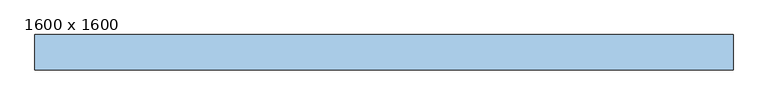
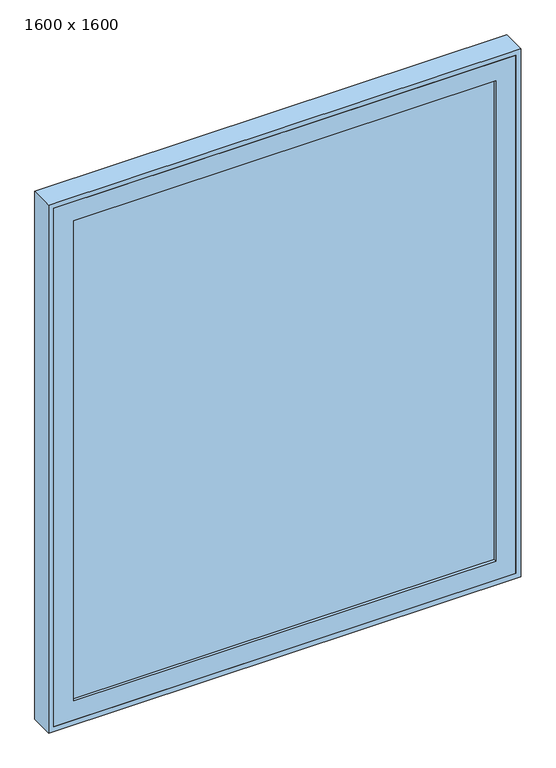
"""IFC4 building model written with IfcOpenShell, lengths in millimetres: window geometry, Aluprof_MB-79N-SI_E_Alu_Window-1sash-FIX_ENG_R-00206 : 1600 x 1600."""

from ifc_helpers import new_model, si_unit, frame, origin, place, context, project, spatial, polyline, outline, extrude, faceted_brep, source, transform, mapped, element, save


def window_1600_x_1600_1d4bee44(model_context):
    return source(origin(), model_context, "Body", "SolidModel", [
        faceted_brep([(-619.5, -58.5, 2315.5), (-619.5, -58.5, 826.5), (-619.5, -45.0, 826.5), (-619.5, -45.0, 2315.5), (-675.0, -45.0, 2371.0), (-675.0, -45.0, 771.0), (-675.0, -115.0, 771.0), (-675.0, -115.0, 2371.0), (619.5, -58.5, 826.5), (619.5, -45.0, 826.5), (675.0, -45.0, 771.0), (675.0, -115.0, 771.0), (619.5, -58.5, 2315.5), (619.5, -45.0, 2315.5), (675.0, -45.0, 2371.0), (675.0, -115.0, 2371.0), (-635.5, -58.5, 2331.5), (-635.5, -58.5, 810.5), (635.5, -58.5, 810.5), (635.5, -58.5, 2331.5), (-635.5, -106.5, 2331.5), (-635.5, -106.5, 810.5), (635.5, -106.5, 810.5), (635.5, -106.5, 2331.5), (-616.5, -106.5, 2312.5), (-616.5, -106.5, 829.5), (616.5, -106.5, 829.5), (616.5, -106.5, 2312.5), (-616.5, -115.0, 2312.5), (-616.5, -115.0, 829.5), (616.5, -115.0, 829.5), (616.5, -115.0, 2312.5)], [[[0, 1, 2, 3]], [[4, 5, 6, 7]], [[1, 8, 9, 2]], [[5, 10, 11, 6]], [[8, 12, 13, 9]], [[10, 14, 15, 11]], [[16, 17, 18, 19], [1, 0, 12, 8]], [[12, 0, 3, 13]], [[5, 4, 14, 10], [3, 2, 9, 13]], [[14, 4, 7, 15]], [[20, 21, 17, 16]], [[21, 22, 18, 17]], [[22, 23, 19, 18]], [[21, 20, 23, 22], [24, 25, 26, 27]], [[23, 20, 16, 19]], [[28, 29, 25, 24]], [[29, 30, 26, 25]], [[30, 31, 27, 26]], [[7, 6, 11, 15], [29, 28, 31, 30]], [[31, 28, 24, 27]]]),
        extrude(outline(polyline([(635.5, -58.5), (635.5, -106.5), (-635.5, -106.5), (-635.5, -58.5), (635.5, -58.5)])), frame((0.0, 0.0, 810.5), z_axis=(0.0, 0.0, 1.0), x_axis=(1.0, 0.0, 0.0)), (0.0, 0.0, 1.0), 1521.0),
        extrude(outline(polyline([(2386.0, -690.0), (756.0, -690.0), (756.0, 690.0), (2386.0, 690.0), (2386.0, -690.0)]), holes=[polyline([(771.0, -675.0), (2371.0, -675.0), (2371.0, 675.0), (771.0, 675.0), (771.0, -675.0)])]), frame((0.0, -115.0, 0.0), z_axis=(0.0, 1.0, 0.0), x_axis=(0.0, 0.0, 1.0)), (0.0, 0.0, 1.0), 70.0),
    ])


if __name__ == "__main__":
    model = new_model("IFC4")
    model_context = context("Model", 3, world=origin())
    ifc_project = project(units=[si_unit("LENGTHUNIT", "METRE", prefix="MILLI")], contexts=[model_context])
    site = spatial("IfcSite", under=ifc_project)
    building = spatial("IfcBuilding", under=site)
    placement = place(None, origin())
    window_1600_x_1600_shape = window_1600_x_1600_1d4bee44(model_context)
    element("IfcWindow", 1, ObjectType="Aluprof_MB-79N-SI_E_Alu_Window-1sash-FIX_ENG_R-00206 : 1600 x 1600", at=placement, inside=building, context=model_context, shape_type="MappedRepresentation", body=[
        mapped(window_1600_x_1600_shape, transform((0.0, 0.0, 0.0), x_axis=(1.0, 0.0, 0.0), y_axis=(0.0, 1.0, 0.0), z_axis=(0.0, 0.0, 1.0))),
    ])
    save(model, "model.ifc")

# Revit data of these elements
# Type "Aluprof_MB-79N-SI_E_Alu_Window-1sash-FIX_ENG_R-00206 : 1600 x 1600"
#   Type Mark = "58"
#   Water resistance = "Class E1950, EN 12208"
#   Uniclass2015Version = "v1.6"
#   Uniclass2015Reference = "Pr_30_59_98_02"
#   Uniclass2015Description = "Aluminium window units"
#   URL = "https://aluprof.eu/"
#   Resistance to wind load = "Class C5, EN 12210"
#   Product page URL = "https://aluprof.eu/architekci/katalog-dla-architektow/systemy-okienno-drzwiowe/mb-79n-si-system-okienno-drzwiowy-z-izolacja-termiczna#/materialy/ogolne-informacje"
#   Operation = "SinglePanel"
#   Opening type = "FIX"
#   NBSReference = "45-25-99/310"
#   NBSDescription = "Aluminium window units"
#   Model = "MB-79N SI"
#   Manufacturer = "ALUPROF S.A."
#   Insert type = "SI"
#   IfcExportType = "NOTDEFINED"
#   IfcExportAs = "IfcWindowType"
#   Glazing construction = "6/16/4/16/6"
#   Description = "Single fixed window"
#   Content of the recyclate in the material = "70.7%"
#   COBie.Type.WarrantyDurationParts = ""
#   COBie.Type.Name = ""
#   COBie.Type.Manufacturer = "ALUPROF SA"
#   COBie.Space.Name = ""
#   COBie.Floor.Name = ""
#   COBie.Facility.Name = ""
#   COBie.CreatedOn = ""
#   COBie.CreatedBy = "aluprof.eu"
#   COBie.Component.WarrantyStartDate = ""
#   COBie.Component.Name = "MB-79N SI"
#   Air permeability = "Class 4, EN 12207"
#   Thermal insulation = 0.6000 W/(m²·K)
#   Sash thickness = 79 mm
#   Rough Width = 1380 mm
#   Rough Height = 1630 mm
#   Mounting space = 15 mm
#   Height = 1600 mm
#   Glazing area = 1.93319 m²
#   Frame thickness = 70 mm
#   Exterior wall face offset = 60 mm
#   Sill Height = 771 mm
#   Width = 1350 mm
#   Warm installation [instance default] = yes
#   Schedule No. [instance default] = 1
#   IsExternal = yes
#   COBie.Type = yes
#   COBie = yes
#   GlazingMaterial = Glass_ALUPROF_Clear
#   FrameMaterial = Träfönster WSP Stockholm
#   BackfillingMaterial = ExpandingFoam_ALUPROF_Yellow
#   Wall Closure = (empty or 0)
# Element 1 (IfcWindow, "Aluprof_MB-79N-SI_E_Alu_Window-1sash-FIX_ENG_R-00206 : 1600 x 1600")
#   Materials on its faces: "Träfönster WSP Stockholm", "ExpandingFoam_ALUPROF_Yellow", "Glass_ALUPROF_Clear"
# Materials
#   "Glass_ALUPROF_Clear": class "Glass", colour RGB 22 81 169, transparency 0.85, Model = "GlazingClear", Manufacturer = "ALUPROF S.A.", URL = "https://aluprof.eu/pl-en", Description = "Glazing", Cost = 0
#   "Träfönster WSP Stockholm": class "Generic", colour RGB 45 25 19, transparency 0, Cost = 0
#   "ExpandingFoam_ALUPROF_Yellow": class "Generic", colour RGB 175 175 60, transparency 0, Model = "ExpandingFoam", Manufacturer = "ALUPROF S.A.", URL = "https://aluprof.eu/pl-en", Description = "Expanding foam", Cost = 0
